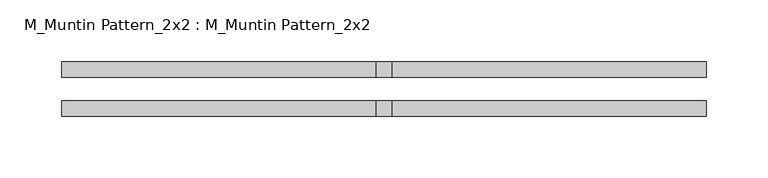
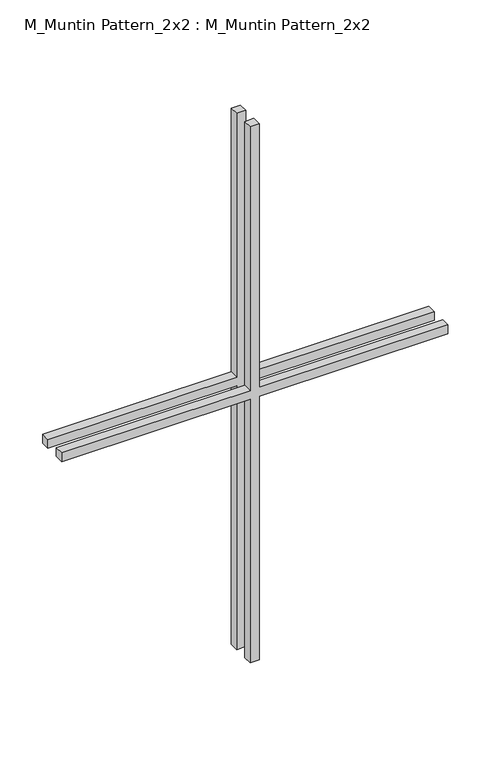
"""IFC4 building model written with IfcOpenShell, lengths in millimetres: proxy geometry, M_Muntin Pattern_2x2 : M_Muntin Pattern_2x2."""

from ifc_helpers import new_model, si_unit, frame, origin, place, context, project, spatial, polyline, outline, extrude, source, transform, mapped, element, save


def m_muntin_pattern_2x2_m_muntin_pattern_2x2_1fb5fae3(model_context):
    return source(origin(), model_context, "Body", "SweptSolid", [
        extrude(outline(polyline([(390.525, -6.35), (390.525, -261.9375), (377.825, -261.9375), (377.825, -6.35), (0.0, -6.35), (0.0, 6.35), (377.825, 6.35), (377.825, 261.9375), (390.525, 261.9375), (390.525, 6.35), (768.35, 6.35), (768.35, -6.35), (390.525, -6.35)])), frame((0.0, -22.225, 0.0), z_axis=(0.0, 1.0, 0.0), x_axis=(0.0, 0.0, 1.0)), (0.0, 0.0, 1.0), 12.7),
        extrude(outline(polyline([(390.525, -6.35), (390.525, -261.9375), (377.825, -261.9375), (377.825, -6.35), (0.0, -6.35), (0.0, 6.35), (377.825, 6.35), (377.825, 261.9375), (390.525, 261.9375), (390.525, 6.35), (768.35, 6.35), (768.35, -6.35), (390.525, -6.35)])), frame((0.0, 9.525, 0.0), z_axis=(0.0, 1.0, 0.0), x_axis=(0.0, 0.0, 1.0)), (0.0, 0.0, 1.0), 12.7),
    ])


if __name__ == "__main__":
    model = new_model("IFC4")
    model_context = context("Model", 3, world=origin())
    ifc_project = project(units=[si_unit("LENGTHUNIT", "METRE", prefix="MILLI")], contexts=[model_context])
    site = spatial("IfcSite", under=ifc_project)
    building = spatial("IfcBuilding", under=site)
    placement = place(None, origin())
    m_muntin_pattern_2x2_m_muntin_pattern_2x2_shape = m_muntin_pattern_2x2_m_muntin_pattern_2x2_1fb5fae3(model_context)
    element("IfcBuildingElementProxy", 1, Name="M_Muntin Pattern_2x2 : M_Muntin Pattern_2x2", ObjectType="M_Muntin Pattern_2x2 : M_Muntin Pattern_2x2", at=placement, inside=building, context=model_context, shape_type="MappedRepresentation", body=[
        mapped(m_muntin_pattern_2x2_m_muntin_pattern_2x2_shape, transform((0.0, 0.0, 0.0), x_axis=(1.0, 0.0, 0.0), y_axis=(0.0, 1.0, 0.0), z_axis=(0.0, 0.0, 1.0))),
    ])
    save(model, "model.ifc")

# Revit data of these elements
# Type "M_Muntin Pattern_2x2 : M_Muntin Pattern_2x2"
#   Width [instance default] = 3' - 11.24409"
#   Thickness = 0' - 0 1/2"
#   Height [instance default] = 3' - 11.24409"
#   Distance = 0' - 0 3/4"
#   Interior Material [instance default] = none
#   Exterior Material [instance default] = none
#   Default Elevation = 0
# Element 1 (IfcBuildingElementProxy, "M_Muntin Pattern_2x2 : M_Muntin Pattern_2x2")
#   Width = 1' - 8 5/8"
#   Height = 2' - 6 1/4"
#   Interior Material = Wood - Stained
#   Exterior Material = Clad - White
#   Materials on its faces: "Clad - White", "Wood - Stained"
# Materials
#   "Clad - White": class "Wood", colour RGB 242 242 238, transparency 0, Cost = 0
#   "Wood - Stained": class "Wood", colour RGB 224 178 126, transparency 0, Cost = 0
